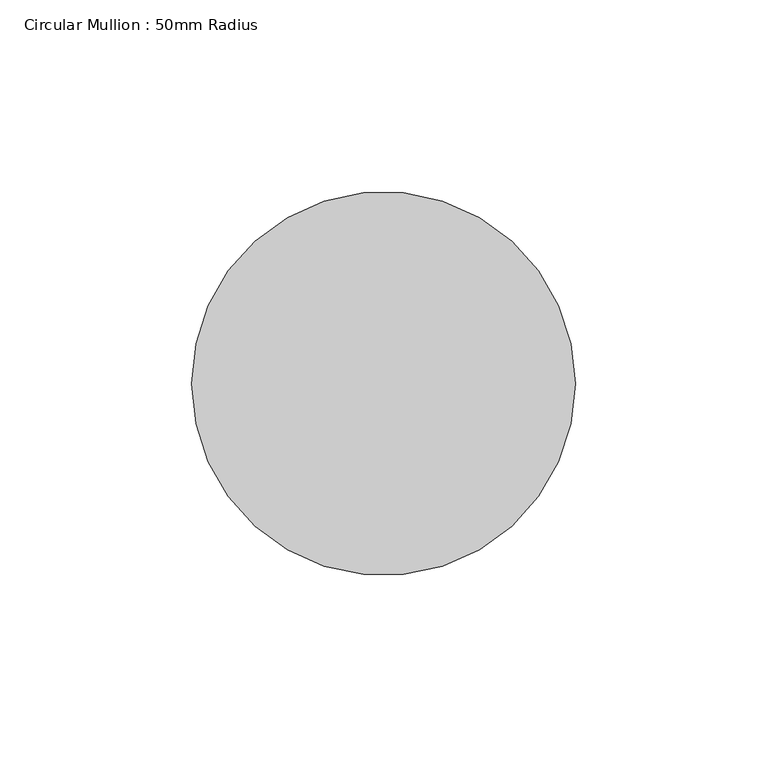
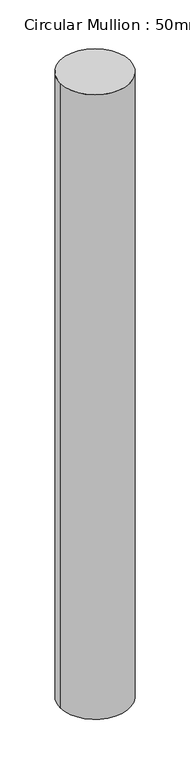
"""IFC4 building model written with IfcOpenShell, lengths in millimetres: member geometry, Circular Mullion : 50mm Radius."""

import ifcopenshell
import ifcopenshell.guid

model = None  # the IFC model being written
_history = None  # IfcOwnerHistory: only IFC2X3 demands one
_inside = {}  # id of a spatial element -> (the spatial element, [elements in it])
_under = {}  # id of a project, library or spatial element -> (it, [spatial elements below it])
_declared = {}  # id of a project -> (the project, [libraries it declares])
_typed = {}  # id of a type object -> (the type object, [elements of that type])
_made_of = {}  # id of a material, layer set ... -> (it, [elements and type objects made of it])


def new_model(schema):
    """Start an empty IFC model of exactly this schema.

    Asked for "IFC4X3", IfcOpenShell would pick the latest addendum, in which some entities
    have other attributes; the version numbers below select the first issue.
    IFC2X3 requires an IfcOwnerHistory on every rooted entity: one is made here for all.
    """
    global model, _history
    if schema == "IFC4X3":
        model = ifcopenshell.file(schema_version=(4, 3, 0, 0))
    else:
        model = ifcopenshell.file(schema=schema)
    _inside.clear()
    _under.clear()
    _declared.clear()
    _typed.clear()
    _made_of.clear()
    _history = None
    if model.schema == "IFC2X3":
        org = make("IfcOrganization", Name="unknown")
        user = make(
            "IfcPersonAndOrganization",
            ThePerson=make("IfcPerson", FamilyName="unknown"),
            TheOrganization=org,
        )
        app = make(
            "IfcApplication",
            ApplicationDeveloper=org,
            Version="unknown",
            ApplicationFullName="unknown",
            ApplicationIdentifier="unknown",
        )
        _history = make(
            "IfcOwnerHistory",
            OwningUser=user,
            OwningApplication=app,
            ChangeAction="ADDED",
            CreationDate=0,
        )
    return model


def make(cls, **values):
    """One entity of the class cls with the attributes given. An attribute that is None is left unset."""
    return model.create_entity(
        cls, **{name: value for name, value in values.items() if value is not None}
    )


def rooted(cls, **values):
    """An entity with a GlobalId (a new one), such as an element, a storey or a relation."""
    return make(cls, GlobalId=ifcopenshell.guid.new(), OwnerHistory=_history, **values)


def si_unit(unit_type, name, prefix=None):
    """IfcSIUnit, for example si_unit("LENGTHUNIT", "METRE", prefix="MILLI")."""
    return make("IfcSIUnit", UnitType=unit_type, Prefix=prefix, Name=name)


def assignment(units):
    """IfcUnitAssignment: the units of a project."""
    return None if units is None else make("IfcUnitAssignment", Units=units)


def point(xyz):
    """IfcCartesianPoint."""
    return None if xyz is None else make("IfcCartesianPoint", Coordinates=xyz)


def direction(xyz):
    """IfcDirection."""
    return None if xyz is None else make("IfcDirection", DirectionRatios=xyz)


def frame(location, z_axis=None, x_axis=None):
    """IfcAxis2Placement3D, a coordinate frame: its origin and axes. An axis left out is left unset."""
    return make(
        "IfcAxis2Placement3D",
        Location=point(location),
        Axis=direction(z_axis),
        RefDirection=direction(x_axis),
    )


def frame_2d(location, x_axis=None):
    """IfcAxis2Placement2D, a coordinate frame in the plane: its origin and x axis."""
    return make(
        "IfcAxis2Placement2D", Location=point(location), RefDirection=direction(x_axis)
    )


def origin():
    """The frame at (0, 0, 0) with its axes left unset."""
    return frame((0.0, 0.0, 0.0))


def origin_2d():
    """The frame at (0, 0) in the plane with its x axis left unset."""
    return frame_2d((0.0, 0.0))


def place(relative_to, where):
    """IfcLocalPlacement: puts the frame where relative to a parent placement (None: the world)."""
    return make(
        "IfcLocalPlacement", PlacementRelTo=relative_to, RelativePlacement=where
    )


def context(
    kind, dimensions, precision=None, world=None, true_north=None, identifier=None
):
    """IfcGeometricRepresentationContext, for example the 3D "Model" context."""
    return make(
        "IfcGeometricRepresentationContext",
        ContextIdentifier=identifier,
        ContextType=kind,
        CoordinateSpaceDimension=dimensions,
        Precision=precision,
        WorldCoordinateSystem=world,
        TrueNorth=true_north,
    )


def project(units=None, contexts=None):
    """IfcProject with its units and contexts."""
    return rooted(
        "IfcProject",
        Name="project",
        RepresentationContexts=contexts,
        UnitsInContext=assignment(units),
    )


def spatial(cls, under=None, at=None, **own):
    """A site, building, storey or space (cls), placed at a placement, below another one or the project."""
    s = rooted(cls, ObjectPlacement=at, **own)
    if under is not None:
        _under.setdefault(under.id(), (under, []))[1].append(s)
    return s


def circle_curve(where, radius):
    """IfcCircle in the frame where."""
    return make("IfcCircle", Position=where, Radius=radius)


def trimmed(basis, trim1, trim2, sense, master):
    """IfcTrimmedCurve: the piece of a basis curve between two trims."""
    return make(
        "IfcTrimmedCurve",
        BasisCurve=basis,
        Trim1=trim1,
        Trim2=trim2,
        SenseAgreement=sense,
        MasterRepresentation=master,
    )


def segment(curve, same_sense, transition):
    """IfcCompositeCurveSegment."""
    return make(
        "IfcCompositeCurveSegment",
        Transition=transition,
        SameSense=same_sense,
        ParentCurve=curve,
    )


def composite_curve(segments, self_intersect=None):
    """IfcCompositeCurve: segments joined end to end."""
    return make("IfcCompositeCurve", Segments=segments, SelfIntersect=self_intersect)


def outline(outer, holes=None, kind="AREA"):
    """IfcArbitraryClosedProfileDef: a profile drawn as a closed curve; with holes, ...WithVoids."""
    if holes is None:
        return make("IfcArbitraryClosedProfileDef", ProfileType=kind, OuterCurve=outer)
    return make(
        "IfcArbitraryProfileDefWithVoids",
        ProfileType=kind,
        OuterCurve=outer,
        InnerCurves=holes,
    )


def extrude(swept, where, along, depth):
    """IfcExtrudedAreaSolid: the profile swept, set in the frame where, extruded along a direction by depth."""
    return make(
        "IfcExtrudedAreaSolid",
        SweptArea=swept,
        Position=where,
        ExtrudedDirection=direction(along),
        Depth=depth,
    )


def shape(context_of_items, identifier, shape_type, items):
    """IfcShapeRepresentation: the items that make up one representation, for example the "Body"."""
    return make(
        "IfcShapeRepresentation",
        ContextOfItems=context_of_items,
        RepresentationIdentifier=identifier,
        RepresentationType=shape_type,
        Items=items,
    )


def source(mapping_origin, context_of_items, identifier, shape_type, items):
    """IfcRepresentationMap: a shape defined once, which mapped items show again and again."""
    return make(
        "IfcRepresentationMap",
        MappingOrigin=mapping_origin,
        MappedRepresentation=shape(context_of_items, identifier, shape_type, items),
    )


def transform(
    local_origin,
    x_axis=None,
    y_axis=None,
    z_axis=None,
    scale=None,
    scale2=None,
    scale3=None,
    uniform=True,
):
    """IfcCartesianTransformationOperator3D, or its non-uniform kind. x_axis, y_axis, z_axis: its Axis1, 2, 3."""
    if uniform:
        return make(
            "IfcCartesianTransformationOperator3D",
            Axis1=direction(x_axis),
            Axis2=direction(y_axis),
            LocalOrigin=point(local_origin),
            Scale=scale,
            Axis3=direction(z_axis),
        )
    return make(
        "IfcCartesianTransformationOperator3DnonUniform",
        Axis1=direction(x_axis),
        Axis2=direction(y_axis),
        LocalOrigin=point(local_origin),
        Scale=scale,
        Axis3=direction(z_axis),
        Scale2=scale2,
        Scale3=scale3,
    )


def mapped(mapping_source, mapping_target):
    """IfcMappedItem: shows the shape of a source again, moved by a transform."""
    return make(
        "IfcMappedItem", MappingSource=mapping_source, MappingTarget=mapping_target
    )


def made_of(thing, what):
    """Note that an element or type object is made of a material, layer set ...; save() writes the relation."""
    if what is not None:
        _made_of.setdefault(what.id(), (what, []))[1].append(thing)
    return thing


def element(
    cls,
    number,
    at=None,
    inside=None,
    cuts=None,
    type_object=None,
    material=None,
    context=None,
    identifier="Body",
    shape_type=None,
    held_by="IfcProductDefinitionShape",
    body=None,
    shapes=None,
    **own,
):
    """One element of the class cls, such as IfcWall. Its Tag is "e" and its number.

    at: its placement. inside: the storey or other place that contains it. cuts: it is an
    opening in that element (IfcRelVoidsElement). A single representation is given by context,
    identifier, shape_type and body (its items); several are given by shapes. held_by: the class
    of the entity that holds the representations. save() writes the other relations.
    """
    e = rooted(cls, Tag="e%d" % number, ObjectPlacement=at, **own)
    if body is not None:
        shapes = [shape(context, identifier, shape_type, body)]
    if shapes is not None:
        e.Representation = make(held_by, Representations=shapes)
    if inside is not None:
        _inside.setdefault(inside.id(), (inside, []))[1].append(e)
    if cuts is not None:
        rooted(
            "IfcRelVoidsElement", RelatingBuildingElement=cuts, RelatedOpeningElement=e
        )
    if type_object is not None:
        _typed.setdefault(type_object.id(), (type_object, []))[1].append(e)
    return made_of(e, material)


def aggregate(whole, parts):
    """IfcRelAggregates: a whole, such as a stair, and the parts it consists of."""
    return rooted("IfcRelAggregates", RelatingObject=whole, RelatedObjects=parts)


def save(model, path):
    """Write the relations noted so far, then the file.

    IfcRelAggregates (storeys below a building ...), IfcRelContainedInSpatialStructure (elements
    in a storey), IfcRelDefinesByType, IfcRelAssociatesMaterial and IfcRelDeclares: one each for
    every whole, place, type object, material and project.
    """
    for whole, parts in _under.values():
        aggregate(whole, parts)
    for where, things in _inside.values():
        rooted(
            "IfcRelContainedInSpatialStructure",
            RelatedElements=things,
            RelatingStructure=where,
        )
    for kind, things in _typed.values():
        rooted("IfcRelDefinesByType", RelatedObjects=things, RelatingType=kind)
    for what, things in _made_of.values():
        rooted("IfcRelAssociatesMaterial", RelatedObjects=things, RelatingMaterial=what)
    for by, libraries in _declared.values():
        rooted("IfcRelDeclares", RelatingContext=by, RelatedDefinitions=libraries)
    model.write(path)


def circular_mullion_50mm_radius_b3cf57fc(model_context):
    return source(origin(), model_context, "Body", "SweptSolid", [
        extrude(outline(composite_curve([segment(trimmed(circle_curve(origin_2d(), 50.0), [point((50.0, 0.0))], [point((-50.0, 0.0))], False, "CARTESIAN"), True, "CONTINUOUS"), segment(trimmed(circle_curve(origin_2d(), 50.0), [point((-50.0, 0.0))], [point((50.0, 0.0))], False, "CARTESIAN"), True, "CONTINUOUS")], self_intersect=False)), frame((0.0, 0.0, -947.100572), z_axis=(0.0, 0.0, 1.0), x_axis=(1.0, 0.0, 0.0)), (0.0, 0.0, 1.0), 947.100572),
    ])


if __name__ == "__main__":
    model = new_model("IFC4")
    model_context = context("Model", 3, world=origin())
    ifc_project = project(units=[si_unit("LENGTHUNIT", "METRE", prefix="MILLI")], contexts=[model_context])
    site = spatial("IfcSite", under=ifc_project)
    building = spatial("IfcBuilding", under=site)
    placement = place(None, origin())
    circular_mullion_50mm_radius_shape = circular_mullion_50mm_radius_b3cf57fc(model_context)
    element("IfcMember", 1, ObjectType="Circular Mullion : 50mm Radius", at=placement, inside=building, context=model_context, shape_type="MappedRepresentation", body=[
        mapped(circular_mullion_50mm_radius_shape, transform((0.0, 0.0, 0.0), x_axis=(1.0, 0.0, 0.0), y_axis=(0.0, 1.0, 0.0), z_axis=(0.0, 0.0, 1.0))),
    ])
    save(model, "model.ifc")

# Revit data of these elements
# Type "Circular Mullion : 50mm Radius"
#   built-in parameter 1007350 = 0.164042 (stored number, unit not read)
# Element 1 (IfcMember, "Circular Mullion : 50mm Radius")
#   Materials on its faces: "Aluminium"
# Materials
#   "Aluminium": class "Metal", colour RGB 247 247 247, transparency 0, Description = "Aluminium 6061", Cost = 0
